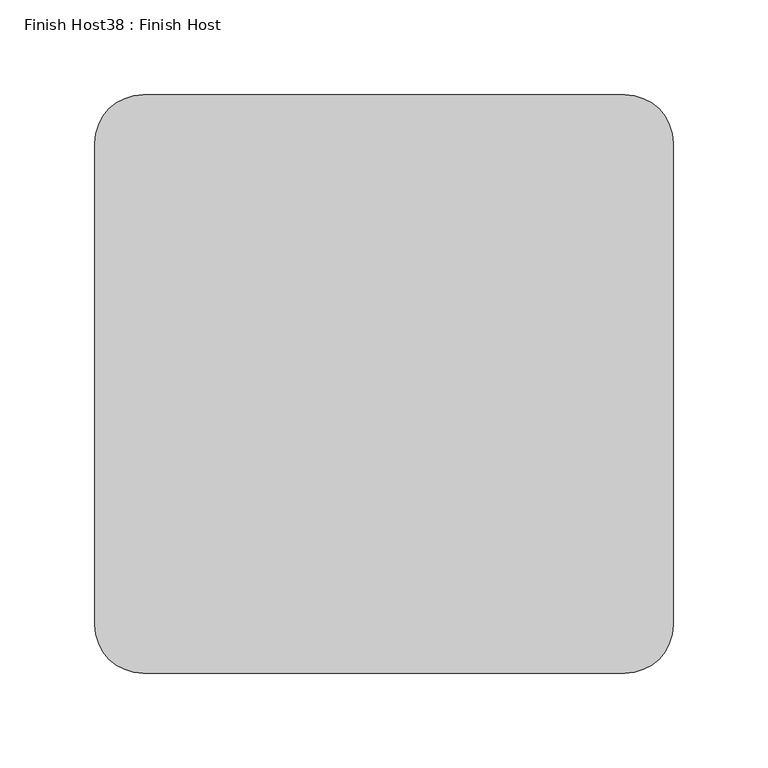
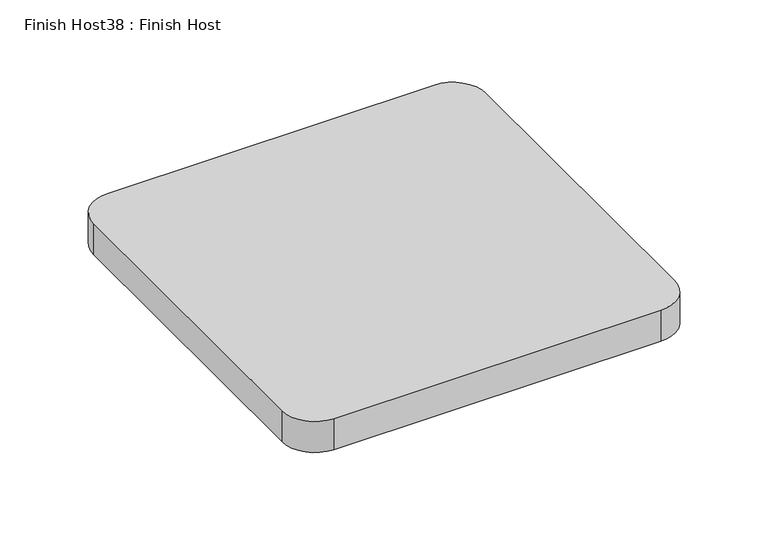
"""IFC4 building model written with IfcOpenShell, lengths in millimetres: proxy geometry, Finish Host38 : Finish Host."""

from ifc_helpers import new_model, si_unit, point, frame_2d, origin, origin_with_axes, place, context, project, spatial, polyline, circle_curve, trimmed, segment, composite_curve, outline, extrude, source, transform, mapped, element, save


def finish_host38_finish_host_f714d161(model_context):
    return source(origin(), model_context, "Body", "SweptSolid", [
        extrude(outline(composite_curve([segment(polyline([(-17113.2939795, 14061.2419385), (-17113.2939795, 14315.2419385)]), True, "CONTINUOUS"), segment(trimmed(circle_curve(frame_2d((-17087.8939795, 14315.2419385)), 25.4), [point((-17113.2939795, 14315.2419385))], [point((-17087.8939795, 14340.6419385))], False, "CARTESIAN"), True, "CONTINUOUS"), segment(polyline([(-17087.8939795, 14340.6419385), (-16833.8939795, 14340.6419385)]), True, "CONTINUOUS"), segment(trimmed(circle_curve(frame_2d((-16833.8939795, 14315.2419385)), 25.4), [point((-16833.8939795, 14340.6419385))], [point((-16808.4939795, 14315.2419385))], False, "CARTESIAN"), True, "CONTINUOUS"), segment(polyline([(-16808.4939795, 14315.2419385), (-16808.4939795, 14061.2419385)]), True, "CONTINUOUS"), segment(trimmed(circle_curve(frame_2d((-16833.8939795, 14061.2419385)), 25.4), [point((-16808.4939795, 14061.2419385))], [point((-16833.8939795, 14035.8419385))], False, "CARTESIAN"), True, "CONTINUOUS"), segment(polyline([(-16833.8939795, 14035.8419385), (-17087.8939795, 14035.8419385)]), True, "CONTINUOUS"), segment(trimmed(circle_curve(frame_2d((-17087.8939795, 14061.2419385)), 25.4), [point((-17087.8939795, 14035.8419385))], [point((-17113.2939795, 14061.2419385))], False, "CARTESIAN"), True, "CONTINUOUS")], self_intersect=False)), origin_with_axes(), (0.0, 0.0, 1.0), 25.4),
    ])


if __name__ == "__main__":
    model = new_model("IFC4")
    model_context = context("Model", 3, world=origin())
    ifc_project = project(units=[si_unit("LENGTHUNIT", "METRE", prefix="MILLI")], contexts=[model_context])
    site = spatial("IfcSite", under=ifc_project)
    building = spatial("IfcBuilding", under=site)
    placement = place(None, origin())
    finish_host38_finish_host_shape = finish_host38_finish_host_f714d161(model_context)
    element("IfcBuildingElementProxy", 1, Name="Finish Host38 : Finish Host", ObjectType="Finish Host38 : Finish Host", at=placement, inside=building, context=model_context, shape_type="MappedRepresentation", body=[
        mapped(finish_host38_finish_host_shape, transform((0.0, 0.0, 0.0), x_axis=(1.0, 0.0, 0.0), y_axis=(0.0, 1.0, 0.0), z_axis=(0.0, 0.0, 1.0))),
    ])
    save(model, "model.ifc")

# Revit data of these elements
# Type "Finish Host38 : Finish Host"
#   Panel Material = none
# Element 1 (IfcBuildingElementProxy, "Finish Host38 : Finish Host")
#   Materials on its faces: "Thread - Teknion - White"
# Materials
#   "Thread - Teknion - White": class "Fabric", colour RGB 203 205 202, transparency 0, Model = "F206", Manufacturer = "Teknion Studio", URL = "http://www.teknion.com/", Description = "Fantasme Full Wool", Cost = 0
